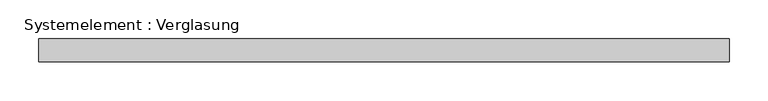
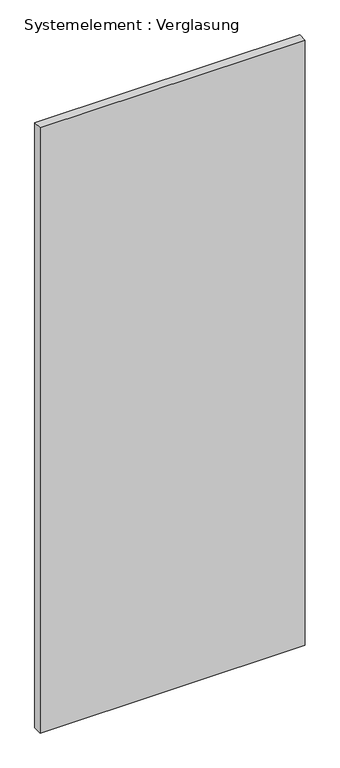
"""IFC4 building model written with IfcOpenShell, lengths in millimetres: plate geometry, Systemelement : Verglasung."""

from ifc_helpers import new_model, si_unit, origin, origin_with_axes, place, context, project, spatial, polyline, outline, extrude, source, transform, mapped, element, save


def systemelement_verglasung_ea6cf5dd(model_context):
    return source(origin(), model_context, "Body", "SweptSolid", [
        extrude(outline(polyline([(447.5113473, -15.0), (-447.5113473, -15.0), (-447.5113473, 15.0), (447.5113473, 15.0), (447.5113473, -15.0)])), origin_with_axes(), (0.0, 0.0, 1.0), 2160.0),
    ])


if __name__ == "__main__":
    model = new_model("IFC4")
    model_context = context("Model", 3, world=origin())
    ifc_project = project(units=[si_unit("LENGTHUNIT", "METRE", prefix="MILLI")], contexts=[model_context])
    site = spatial("IfcSite", under=ifc_project)
    building = spatial("IfcBuilding", under=site)
    placement = place(None, origin())
    systemelement_verglasung_shape = systemelement_verglasung_ea6cf5dd(model_context)
    element("IfcPlate", 1, ObjectType="Systemelement : Verglasung", at=placement, inside=building, context=model_context, shape_type="MappedRepresentation", body=[
        mapped(systemelement_verglasung_shape, transform((0.0, 0.0, 0.0), x_axis=(1.0, 0.0, 0.0), y_axis=(0.0, 1.0, 0.0), z_axis=(0.0, 0.0, 1.0))),
    ])
    save(model, "model.ifc")

# Revit data of these elements
# Type "Systemelement : Verglasung"
#   Construction Type Id = "GSP4R"
#   Analytic Construction = "1/8 Zoll Pilkington-Verglasung einfach"
#   Visual Light Transmittance = 0.9
#   Solar Heat Gain Coefficient = 0.86
#   Heat Transfer Coefficient (U) = 6.7069 W/(m²·K)
# Element 1 (IfcPlate, "Systemelement : Verglasung")
#   Materials on its faces: "Glas"
# Materials
#   "Glas": class "Glas", colour RGB 0 0 255, transparency 0.75, Comments = "Render-Darstellung nicht aktualisiert ", Cost = 0
